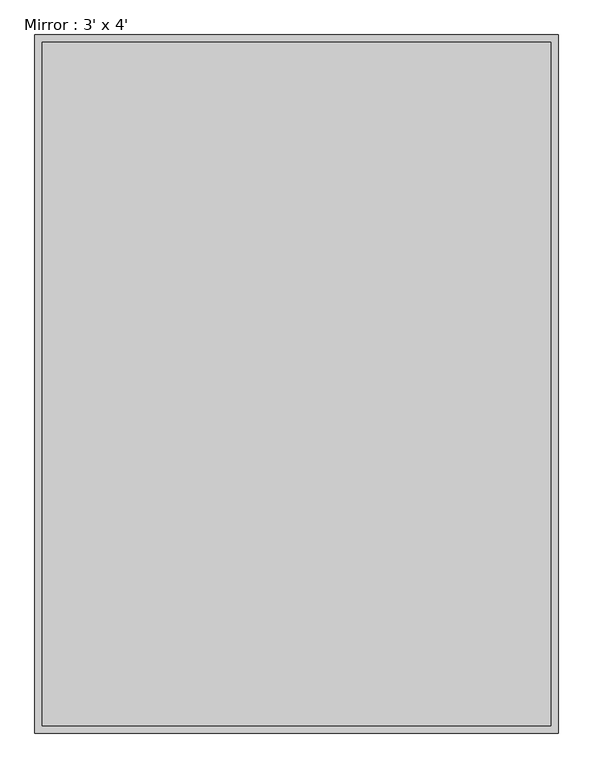
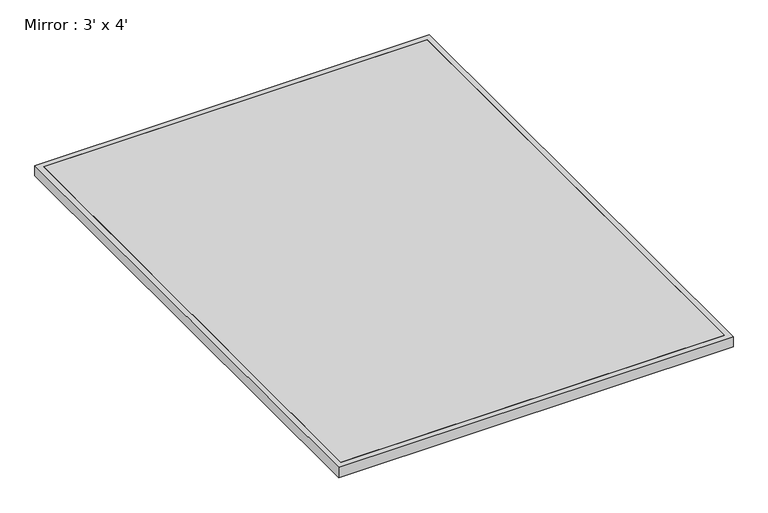
"""IFC4 building model written with IfcOpenShell, lengths in millimetres: furniture geometry, Mirror : 3' x 4'."""

from ifc_helpers import new_model, si_unit, origin, origin_with_axes, place, context, project, spatial, polyline, outline, extrude, source, transform, mapped, element, save


def mirror_3_x_4_424c4327(model_context):
    return source(origin(), model_context, "Body", "SweptSolid", [
        extrude(outline(polyline([(444.5, -596.9), (-444.5, -596.9), (-444.5, 596.9), (444.5, 596.9), (444.5, -596.9)])), origin_with_axes(), (0.0, 0.0, 1.0), 25.4),
        extrude(outline(polyline([(457.2, -609.6), (-457.2, -609.6), (-457.2, 609.6), (457.2, 609.6), (457.2, -609.6)]), holes=[polyline([(444.5, -596.9), (444.5, 596.9), (-444.5, 596.9), (-444.5, -596.9), (444.5, -596.9)])]), origin_with_axes(), (0.0, 0.0, 1.0), 25.4),
    ])


if __name__ == "__main__":
    model = new_model("IFC4")
    model_context = context("Model", 3, world=origin())
    ifc_project = project(units=[si_unit("LENGTHUNIT", "METRE", prefix="MILLI")], contexts=[model_context])
    site = spatial("IfcSite", under=ifc_project)
    building = spatial("IfcBuilding", under=site)
    placement = place(None, origin())
    mirror_3_x_4_shape = mirror_3_x_4_424c4327(model_context)
    element("IfcFurniture", 1, ObjectType="Mirror : 3' x 4'", at=placement, inside=building, context=model_context, shape_type="MappedRepresentation", body=[
        mapped(mirror_3_x_4_shape, transform((0.0, 0.0, 0.0), x_axis=(1.0, 0.0, 0.0), y_axis=(0.0, 1.0, 0.0), z_axis=(0.0, 0.0, 1.0))),
    ])
    save(model, "model.ifc")

# Revit data of these elements
# Type "Mirror : 3' x 4'"
#   Width = 3' - 0"
#   Height = 4' - 0"
#   Frame Thickness = 0' - 0 1/2"
#   Default Elevation = 4' - 0"
#   Mirror = Glass - Mirror
#   Frame = Metal - Chrome
# Element 1 (IfcFurniture, "Mirror : 3' x 4'")
#   Materials on its faces: "Metal - Chrome", "Glass - Mirror"
# Materials
#   "Glass - Mirror": class "Glass", colour RGB 0 128 192, transparency 0.75, Comments = "Rendering appearance not upgraded Rendering appearance not upgraded ", Description = "Glass"
#   "Metal - Chrome": class "Metal", colour RGB 244 244 244, transparency 0, Comments = "Rendering appearance not upgraded Rendering appearance not upgraded ", Description = "Chrome"
